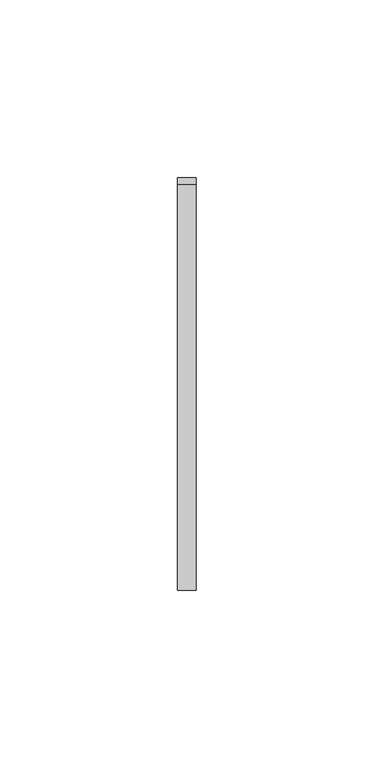
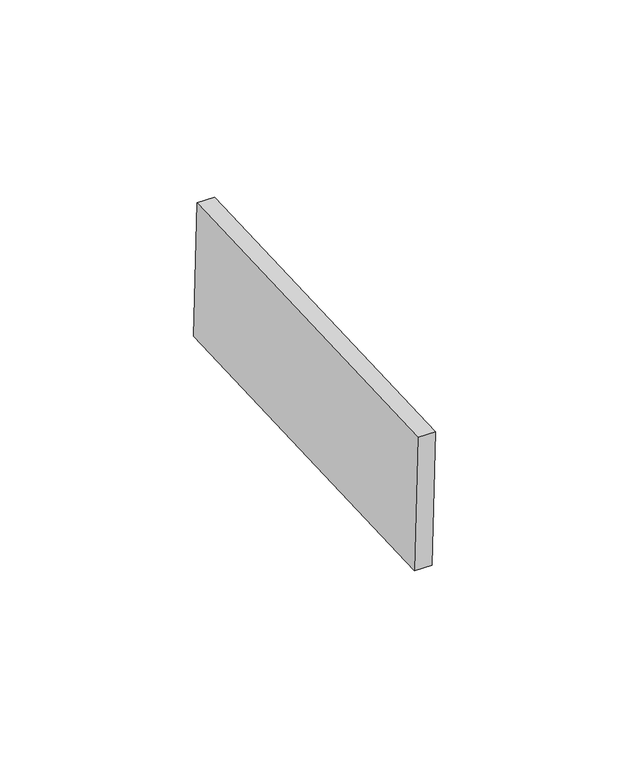
"""IFC4 building model written with IfcOpenShell, lengths in millimetres: proxy geometry, Inner panel:Inner panel:1:Inner panel:1 : Inner panel:Inner panel:300324:2:Inner panel:1:Inner panel:1 : Inner panel:Inner panel:300324:2 : Inner panel:Inner panel:1:Inner panel:1 : Inner panel:Inner panel:300324:300043:80 : Inner panel:Inner panel:1:Inner panel:1 : Inner panel:Inner panel:300324:2:Inner panel:1:Inner panel:1 : Inner panel:Inner panel:300324:2 : Inner panel:Inner panel:1:Inner panel:1 : Inner panel:Inner panel:300324:300043:308120."""

from ifc_helpers import new_model, si_unit, frame, origin, place, context, project, spatial, polyline, outline, extrude, source, transform, mapped, element, save


def generic_models_d6ff326d(model_context):
    return source(origin(), model_context, "Body", "SweptSolid", [
        extrude(outline(polyline([(0.0, -114.3), (0.0, 0.0), (5.2138089, 0.0), (5.2138089, -114.3), (0.0, -114.3)])), frame((593123.795117, -577458.3096573, 4016.6427799), z_axis=(0.0, -0.04163054471216399, 0.9991330730923527), x_axis=(-1.0, 0.0, 0.0)), (0.0, 0.0, 1.0), 43.2233908),
    ])


if __name__ == "__main__":
    model = new_model("IFC4")
    model_context = context("Model", 3, world=origin())
    ifc_project = project(units=[si_unit("LENGTHUNIT", "METRE", prefix="MILLI")], contexts=[model_context])
    site = spatial("IfcSite", under=ifc_project)
    building = spatial("IfcBuilding", under=site)
    placement = place(None, origin())
    generic_models_shape = generic_models_d6ff326d(model_context)
    element("IfcBuildingElementProxy", 1, Name="Inner panel:Inner panel:1:Inner panel:1 : Inner panel:Inner panel:300324:2:Inner panel:1:Inner panel:1 : Inner panel:Inner panel:300324:2 : Inner panel:Inner panel:1:Inner panel:1 : Inner panel:Inner panel:300324:300043:80 : Inner panel:Inner panel:1:Inner panel:1 : Inner panel:Inner panel:300324:2:Inner panel:1:Inner panel:1 : Inner panel:Inner panel:300324:2 : Inner panel:Inner panel:1:Inner panel:1 : Inner panel:Inner panel:300324:300043:308120", ObjectType="Inner panel:Inner panel:1:Inner panel:1 : Inner panel:Inner panel:300324:2:Inner panel:1:Inner panel:1 : Inner panel:Inner panel:300324:2 : Inner panel:Inner panel:1:Inner panel:1 : Inner panel:Inner panel:300324:300043:80 : Inner panel:Inner panel:1:Inner panel:1 : Inner panel:Inner panel:300324:2:Inner panel:1:Inner panel:1 : Inner panel:Inner panel:300324:2 : Inner panel:Inner panel:1:Inner panel:1 : Inner panel:Inner panel:300324:300043:308120", at=placement, inside=building, context=model_context, shape_type="MappedRepresentation", body=[
        mapped(generic_models_shape, transform((0.0, 0.0, 0.0), x_axis=(1.0, 0.0, 0.0), y_axis=(0.0, 1.0, 0.0), z_axis=(0.0, 0.0, 1.0))),
    ])
    save(model, "model.ifc")

# Revit data of these elements
# Type "Inner panel:Inner panel:1:Inner panel:1 : Inner panel:Inner panel:300324:2:Inner panel:1:Inner panel:1 : Inner panel:Inner panel:300324:2 : Inner panel:Inner panel:1:Inner panel:1 : Inner panel:Inner panel:300324:300043:80 : Inner panel:Inner panel:1:Inner panel:1 : Inner panel:Inner panel:300324:2:Inner panel:1:Inner panel:1 : Inner panel:Inner panel:300324:2 : Inner panel:Inner panel:1:Inner panel:1 : Inner panel:Inner panel:300324:300043:308120"
#   NameOverride = "Inner panel:Inner panel:1:Inner panel:1 : Inner panel:Inner panel:300324:2:Inner panel:1:Inner panel:1 : Inner panel:Inner panel:300324:2 : Inner panel:Inner panel:1:Inner panel:1 : Inner panel:Inner panel:300324:300043:308120"
#   ObjectTypeOverride = "Inner panel:1:Inner panel:1 : Inner panel:Inner panel:300324:2 : Inner panel:Inner panel:1:Inner panel:1 : Inner panel:Inner panel:300324:300043"
#   Reference = "Inner panel"
#   Tag = "308120"
# Element 1 (IfcBuildingElementProxy, "Inner panel:Inner panel:1:Inner panel:1 : Inner panel:Inner panel:300324:2:Inner panel:1:Inner panel:1 : Inner panel:Inner panel:300324:2 : Inner panel:Inner panel:1:Inner panel:1 : Inner panel:Inner panel:300324:300043:80 : Inner panel:Inner panel:1:Inner panel:1 : Inner panel:Inner panel:300324:2:Inner panel:1:Inner panel:1 : Inner panel:Inner panel:300324:2 : Inner panel:Inner panel:1:Inner panel:1 : Inner panel:Inner panel:300324:300043:308120")
#   Materials on its faces: "SLIDING CLIP"
# Materials
#   "SLIDING CLIP": class "Generic", colour RGB 120 120 120, transparency 0, Cost = 0
